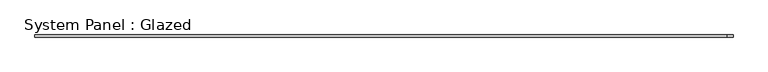
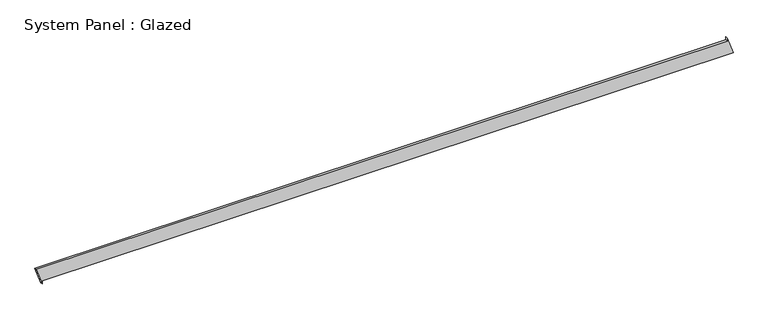
"""IFC4 building model written with IfcOpenShell, lengths in millimetres: plate geometry, System Panel : Glazed."""

import ifcopenshell
import ifcopenshell.guid

model = None  # the IFC model being written
_history = None  # IfcOwnerHistory: only IFC2X3 demands one
_inside = {}  # id of a spatial element -> (the spatial element, [elements in it])
_under = {}  # id of a project, library or spatial element -> (it, [spatial elements below it])
_declared = {}  # id of a project -> (the project, [libraries it declares])
_typed = {}  # id of a type object -> (the type object, [elements of that type])
_made_of = {}  # id of a material, layer set ... -> (it, [elements and type objects made of it])


def new_model(schema):
    """Start an empty IFC model of exactly this schema.

    Asked for "IFC4X3", IfcOpenShell would pick the latest addendum, in which some entities
    have other attributes; the version numbers below select the first issue.
    IFC2X3 requires an IfcOwnerHistory on every rooted entity: one is made here for all.
    """
    global model, _history
    if schema == "IFC4X3":
        model = ifcopenshell.file(schema_version=(4, 3, 0, 0))
    else:
        model = ifcopenshell.file(schema=schema)
    _inside.clear()
    _under.clear()
    _declared.clear()
    _typed.clear()
    _made_of.clear()
    _history = None
    if model.schema == "IFC2X3":
        org = make("IfcOrganization", Name="unknown")
        user = make(
            "IfcPersonAndOrganization",
            ThePerson=make("IfcPerson", FamilyName="unknown"),
            TheOrganization=org,
        )
        app = make(
            "IfcApplication",
            ApplicationDeveloper=org,
            Version="unknown",
            ApplicationFullName="unknown",
            ApplicationIdentifier="unknown",
        )
        _history = make(
            "IfcOwnerHistory",
            OwningUser=user,
            OwningApplication=app,
            ChangeAction="ADDED",
            CreationDate=0,
        )
    return model


def make(cls, **values):
    """One entity of the class cls with the attributes given. An attribute that is None is left unset."""
    return model.create_entity(
        cls, **{name: value for name, value in values.items() if value is not None}
    )


def rooted(cls, **values):
    """An entity with a GlobalId (a new one), such as an element, a storey or a relation."""
    return make(cls, GlobalId=ifcopenshell.guid.new(), OwnerHistory=_history, **values)


def si_unit(unit_type, name, prefix=None):
    """IfcSIUnit, for example si_unit("LENGTHUNIT", "METRE", prefix="MILLI")."""
    return make("IfcSIUnit", UnitType=unit_type, Prefix=prefix, Name=name)


def assignment(units):
    """IfcUnitAssignment: the units of a project."""
    return None if units is None else make("IfcUnitAssignment", Units=units)


def point(xyz):
    """IfcCartesianPoint."""
    return None if xyz is None else make("IfcCartesianPoint", Coordinates=xyz)


def direction(xyz):
    """IfcDirection."""
    return None if xyz is None else make("IfcDirection", DirectionRatios=xyz)


def frame(location, z_axis=None, x_axis=None):
    """IfcAxis2Placement3D, a coordinate frame: its origin and axes. An axis left out is left unset."""
    return make(
        "IfcAxis2Placement3D",
        Location=point(location),
        Axis=direction(z_axis),
        RefDirection=direction(x_axis),
    )


def origin():
    """The frame at (0, 0, 0) with its axes left unset."""
    return frame((0.0, 0.0, 0.0))


def place(relative_to, where):
    """IfcLocalPlacement: puts the frame where relative to a parent placement (None: the world)."""
    return make(
        "IfcLocalPlacement", PlacementRelTo=relative_to, RelativePlacement=where
    )


def context(
    kind, dimensions, precision=None, world=None, true_north=None, identifier=None
):
    """IfcGeometricRepresentationContext, for example the 3D "Model" context."""
    return make(
        "IfcGeometricRepresentationContext",
        ContextIdentifier=identifier,
        ContextType=kind,
        CoordinateSpaceDimension=dimensions,
        Precision=precision,
        WorldCoordinateSystem=world,
        TrueNorth=true_north,
    )


def project(units=None, contexts=None):
    """IfcProject with its units and contexts."""
    return rooted(
        "IfcProject",
        Name="project",
        RepresentationContexts=contexts,
        UnitsInContext=assignment(units),
    )


def spatial(cls, under=None, at=None, **own):
    """A site, building, storey or space (cls), placed at a placement, below another one or the project."""
    s = rooted(cls, ObjectPlacement=at, **own)
    if under is not None:
        _under.setdefault(under.id(), (under, []))[1].append(s)
    return s


def polyline(points):
    """IfcPolyline through the points."""
    return make("IfcPolyline", Points=[point(p) for p in points])


def outline(outer, holes=None, kind="AREA"):
    """IfcArbitraryClosedProfileDef: a profile drawn as a closed curve; with holes, ...WithVoids."""
    if holes is None:
        return make("IfcArbitraryClosedProfileDef", ProfileType=kind, OuterCurve=outer)
    return make(
        "IfcArbitraryProfileDefWithVoids",
        ProfileType=kind,
        OuterCurve=outer,
        InnerCurves=holes,
    )


def extrude(swept, where, along, depth):
    """IfcExtrudedAreaSolid: the profile swept, set in the frame where, extruded along a direction by depth."""
    return make(
        "IfcExtrudedAreaSolid",
        SweptArea=swept,
        Position=where,
        ExtrudedDirection=direction(along),
        Depth=depth,
    )


def shape(context_of_items, identifier, shape_type, items):
    """IfcShapeRepresentation: the items that make up one representation, for example the "Body"."""
    return make(
        "IfcShapeRepresentation",
        ContextOfItems=context_of_items,
        RepresentationIdentifier=identifier,
        RepresentationType=shape_type,
        Items=items,
    )


def source(mapping_origin, context_of_items, identifier, shape_type, items):
    """IfcRepresentationMap: a shape defined once, which mapped items show again and again."""
    return make(
        "IfcRepresentationMap",
        MappingOrigin=mapping_origin,
        MappedRepresentation=shape(context_of_items, identifier, shape_type, items),
    )


def transform(
    local_origin,
    x_axis=None,
    y_axis=None,
    z_axis=None,
    scale=None,
    scale2=None,
    scale3=None,
    uniform=True,
):
    """IfcCartesianTransformationOperator3D, or its non-uniform kind. x_axis, y_axis, z_axis: its Axis1, 2, 3."""
    if uniform:
        return make(
            "IfcCartesianTransformationOperator3D",
            Axis1=direction(x_axis),
            Axis2=direction(y_axis),
            LocalOrigin=point(local_origin),
            Scale=scale,
            Axis3=direction(z_axis),
        )
    return make(
        "IfcCartesianTransformationOperator3DnonUniform",
        Axis1=direction(x_axis),
        Axis2=direction(y_axis),
        LocalOrigin=point(local_origin),
        Scale=scale,
        Axis3=direction(z_axis),
        Scale2=scale2,
        Scale3=scale3,
    )


def mapped(mapping_source, mapping_target):
    """IfcMappedItem: shows the shape of a source again, moved by a transform."""
    return make(
        "IfcMappedItem", MappingSource=mapping_source, MappingTarget=mapping_target
    )


def made_of(thing, what):
    """Note that an element or type object is made of a material, layer set ...; save() writes the relation."""
    if what is not None:
        _made_of.setdefault(what.id(), (what, []))[1].append(thing)
    return thing


def element(
    cls,
    number,
    at=None,
    inside=None,
    cuts=None,
    type_object=None,
    material=None,
    context=None,
    identifier="Body",
    shape_type=None,
    held_by="IfcProductDefinitionShape",
    body=None,
    shapes=None,
    **own,
):
    """One element of the class cls, such as IfcWall. Its Tag is "e" and its number.

    at: its placement. inside: the storey or other place that contains it. cuts: it is an
    opening in that element (IfcRelVoidsElement). A single representation is given by context,
    identifier, shape_type and body (its items); several are given by shapes. held_by: the class
    of the entity that holds the representations. save() writes the other relations.
    """
    e = rooted(cls, Tag="e%d" % number, ObjectPlacement=at, **own)
    if body is not None:
        shapes = [shape(context, identifier, shape_type, body)]
    if shapes is not None:
        e.Representation = make(held_by, Representations=shapes)
    if inside is not None:
        _inside.setdefault(inside.id(), (inside, []))[1].append(e)
    if cuts is not None:
        rooted(
            "IfcRelVoidsElement", RelatingBuildingElement=cuts, RelatedOpeningElement=e
        )
    if type_object is not None:
        _typed.setdefault(type_object.id(), (type_object, []))[1].append(e)
    return made_of(e, material)


def aggregate(whole, parts):
    """IfcRelAggregates: a whole, such as a stair, and the parts it consists of."""
    return rooted("IfcRelAggregates", RelatingObject=whole, RelatedObjects=parts)


def save(model, path):
    """Write the relations noted so far, then the file.

    IfcRelAggregates (storeys below a building ...), IfcRelContainedInSpatialStructure (elements
    in a storey), IfcRelDefinesByType, IfcRelAssociatesMaterial and IfcRelDeclares: one each for
    every whole, place, type object, material and project.
    """
    for whole, parts in _under.values():
        aggregate(whole, parts)
    for where, things in _inside.values():
        rooted(
            "IfcRelContainedInSpatialStructure",
            RelatedElements=things,
            RelatingStructure=where,
        )
    for kind, things in _typed.values():
        rooted("IfcRelDefinesByType", RelatedObjects=things, RelatingType=kind)
    for what, things in _made_of.values():
        rooted("IfcRelAssociatesMaterial", RelatedObjects=things, RelatingMaterial=what)
    for by, libraries in _declared.values():
        rooted("IfcRelDeclares", RelatingContext=by, RelatedDefinitions=libraries)
    model.write(path)


def system_panel_glazed_9d255483(model_context):
    return source(origin(), model_context, "Body", "SweptSolid", [
        extrude(outline(polyline([(0.0, -3958.9104535), (35.3553391, -3958.9104535), (35.3553391, 4027.9323725), (235.7126054, 3959.1507422), (200.3572664, 3959.151181), (200.2581216, -4027.9323725), (0.0, -3958.9104535)])), frame((0.0, -49.5, 0.0), z_axis=(0.0, 1.0, 0.0), x_axis=(0.0, 0.0, 1.0)), (0.0, 0.0, 1.0), 25.0),
    ])


if __name__ == "__main__":
    model = new_model("IFC4")
    model_context = context("Model", 3, world=origin())
    ifc_project = project(units=[si_unit("LENGTHUNIT", "METRE", prefix="MILLI")], contexts=[model_context])
    site = spatial("IfcSite", under=ifc_project)
    building = spatial("IfcBuilding", under=site)
    placement = place(None, origin())
    system_panel_glazed_shape = system_panel_glazed_9d255483(model_context)
    element("IfcPlate", 1, ObjectType="System Panel : Glazed", at=placement, inside=building, context=model_context, shape_type="MappedRepresentation", body=[
        mapped(system_panel_glazed_shape, transform((0.0, 0.0, 0.0), x_axis=(1.0, 0.0, 0.0), y_axis=(0.0, 1.0, 0.0), z_axis=(0.0, 0.0, 1.0))),
    ])
    save(model, "model.ifc")

# Revit data of these elements
# Element 1 (IfcPlate, "System Panel : Glazed")
#   Materials on its faces: "Glass"
# Materials
#   "Glass": class "Glass", colour RGB 218 227 224, transparency 0.85, Description = "Soda Lime Glass", Cost = 0
